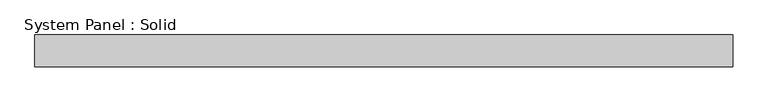
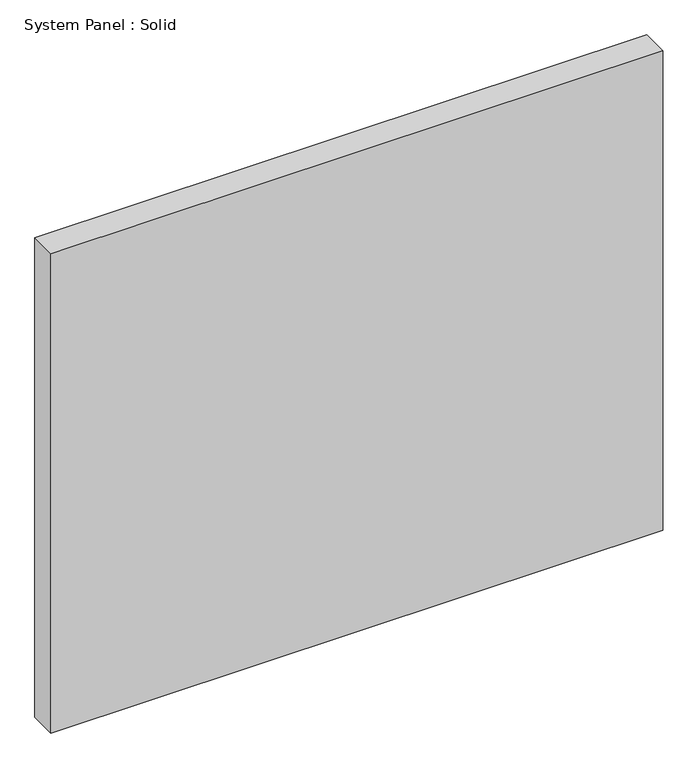
"""IFC4 building model written with IfcOpenShell, lengths in millimetres: plate geometry, System Panel : Solid."""

import ifcopenshell
import ifcopenshell.guid

model = None  # the IFC model being written
_history = None  # IfcOwnerHistory: only IFC2X3 demands one
_inside = {}  # id of a spatial element -> (the spatial element, [elements in it])
_under = {}  # id of a project, library or spatial element -> (it, [spatial elements below it])
_declared = {}  # id of a project -> (the project, [libraries it declares])
_typed = {}  # id of a type object -> (the type object, [elements of that type])
_made_of = {}  # id of a material, layer set ... -> (it, [elements and type objects made of it])


def new_model(schema):
    """Start an empty IFC model of exactly this schema.

    Asked for "IFC4X3", IfcOpenShell would pick the latest addendum, in which some entities
    have other attributes; the version numbers below select the first issue.
    IFC2X3 requires an IfcOwnerHistory on every rooted entity: one is made here for all.
    """
    global model, _history
    if schema == "IFC4X3":
        model = ifcopenshell.file(schema_version=(4, 3, 0, 0))
    else:
        model = ifcopenshell.file(schema=schema)
    _inside.clear()
    _under.clear()
    _declared.clear()
    _typed.clear()
    _made_of.clear()
    _history = None
    if model.schema == "IFC2X3":
        org = make("IfcOrganization", Name="unknown")
        user = make(
            "IfcPersonAndOrganization",
            ThePerson=make("IfcPerson", FamilyName="unknown"),
            TheOrganization=org,
        )
        app = make(
            "IfcApplication",
            ApplicationDeveloper=org,
            Version="unknown",
            ApplicationFullName="unknown",
            ApplicationIdentifier="unknown",
        )
        _history = make(
            "IfcOwnerHistory",
            OwningUser=user,
            OwningApplication=app,
            ChangeAction="ADDED",
            CreationDate=0,
        )
    return model


def make(cls, **values):
    """One entity of the class cls with the attributes given. An attribute that is None is left unset."""
    return model.create_entity(
        cls, **{name: value for name, value in values.items() if value is not None}
    )


def rooted(cls, **values):
    """An entity with a GlobalId (a new one), such as an element, a storey or a relation."""
    return make(cls, GlobalId=ifcopenshell.guid.new(), OwnerHistory=_history, **values)


def si_unit(unit_type, name, prefix=None):
    """IfcSIUnit, for example si_unit("LENGTHUNIT", "METRE", prefix="MILLI")."""
    return make("IfcSIUnit", UnitType=unit_type, Prefix=prefix, Name=name)


def assignment(units):
    """IfcUnitAssignment: the units of a project."""
    return None if units is None else make("IfcUnitAssignment", Units=units)


def point(xyz):
    """IfcCartesianPoint."""
    return None if xyz is None else make("IfcCartesianPoint", Coordinates=xyz)


def direction(xyz):
    """IfcDirection."""
    return None if xyz is None else make("IfcDirection", DirectionRatios=xyz)


def frame(location, z_axis=None, x_axis=None):
    """IfcAxis2Placement3D, a coordinate frame: its origin and axes. An axis left out is left unset."""
    return make(
        "IfcAxis2Placement3D",
        Location=point(location),
        Axis=direction(z_axis),
        RefDirection=direction(x_axis),
    )


def origin():
    """The frame at (0, 0, 0) with its axes left unset."""
    return frame((0.0, 0.0, 0.0))


def origin_with_axes():
    """The frame at (0, 0, 0) with the z axis (0, 0, 1) and the x axis (1, 0, 0) written out."""
    return frame((0.0, 0.0, 0.0), z_axis=(0.0, 0.0, 1.0), x_axis=(1.0, 0.0, 0.0))


def place(relative_to, where):
    """IfcLocalPlacement: puts the frame where relative to a parent placement (None: the world)."""
    return make(
        "IfcLocalPlacement", PlacementRelTo=relative_to, RelativePlacement=where
    )


def context(
    kind, dimensions, precision=None, world=None, true_north=None, identifier=None
):
    """IfcGeometricRepresentationContext, for example the 3D "Model" context."""
    return make(
        "IfcGeometricRepresentationContext",
        ContextIdentifier=identifier,
        ContextType=kind,
        CoordinateSpaceDimension=dimensions,
        Precision=precision,
        WorldCoordinateSystem=world,
        TrueNorth=true_north,
    )


def project(units=None, contexts=None):
    """IfcProject with its units and contexts."""
    return rooted(
        "IfcProject",
        Name="project",
        RepresentationContexts=contexts,
        UnitsInContext=assignment(units),
    )


def spatial(cls, under=None, at=None, **own):
    """A site, building, storey or space (cls), placed at a placement, below another one or the project."""
    s = rooted(cls, ObjectPlacement=at, **own)
    if under is not None:
        _under.setdefault(under.id(), (under, []))[1].append(s)
    return s


def polyline(points):
    """IfcPolyline through the points."""
    return make("IfcPolyline", Points=[point(p) for p in points])


def outline(outer, holes=None, kind="AREA"):
    """IfcArbitraryClosedProfileDef: a profile drawn as a closed curve; with holes, ...WithVoids."""
    if holes is None:
        return make("IfcArbitraryClosedProfileDef", ProfileType=kind, OuterCurve=outer)
    return make(
        "IfcArbitraryProfileDefWithVoids",
        ProfileType=kind,
        OuterCurve=outer,
        InnerCurves=holes,
    )


def extrude(swept, where, along, depth):
    """IfcExtrudedAreaSolid: the profile swept, set in the frame where, extruded along a direction by depth."""
    return make(
        "IfcExtrudedAreaSolid",
        SweptArea=swept,
        Position=where,
        ExtrudedDirection=direction(along),
        Depth=depth,
    )


def shape(context_of_items, identifier, shape_type, items):
    """IfcShapeRepresentation: the items that make up one representation, for example the "Body"."""
    return make(
        "IfcShapeRepresentation",
        ContextOfItems=context_of_items,
        RepresentationIdentifier=identifier,
        RepresentationType=shape_type,
        Items=items,
    )


def source(mapping_origin, context_of_items, identifier, shape_type, items):
    """IfcRepresentationMap: a shape defined once, which mapped items show again and again."""
    return make(
        "IfcRepresentationMap",
        MappingOrigin=mapping_origin,
        MappedRepresentation=shape(context_of_items, identifier, shape_type, items),
    )


def transform(
    local_origin,
    x_axis=None,
    y_axis=None,
    z_axis=None,
    scale=None,
    scale2=None,
    scale3=None,
    uniform=True,
):
    """IfcCartesianTransformationOperator3D, or its non-uniform kind. x_axis, y_axis, z_axis: its Axis1, 2, 3."""
    if uniform:
        return make(
            "IfcCartesianTransformationOperator3D",
            Axis1=direction(x_axis),
            Axis2=direction(y_axis),
            LocalOrigin=point(local_origin),
            Scale=scale,
            Axis3=direction(z_axis),
        )
    return make(
        "IfcCartesianTransformationOperator3DnonUniform",
        Axis1=direction(x_axis),
        Axis2=direction(y_axis),
        LocalOrigin=point(local_origin),
        Scale=scale,
        Axis3=direction(z_axis),
        Scale2=scale2,
        Scale3=scale3,
    )


def mapped(mapping_source, mapping_target):
    """IfcMappedItem: shows the shape of a source again, moved by a transform."""
    return make(
        "IfcMappedItem", MappingSource=mapping_source, MappingTarget=mapping_target
    )


def made_of(thing, what):
    """Note that an element or type object is made of a material, layer set ...; save() writes the relation."""
    if what is not None:
        _made_of.setdefault(what.id(), (what, []))[1].append(thing)
    return thing


def element(
    cls,
    number,
    at=None,
    inside=None,
    cuts=None,
    type_object=None,
    material=None,
    context=None,
    identifier="Body",
    shape_type=None,
    held_by="IfcProductDefinitionShape",
    body=None,
    shapes=None,
    **own,
):
    """One element of the class cls, such as IfcWall. Its Tag is "e" and its number.

    at: its placement. inside: the storey or other place that contains it. cuts: it is an
    opening in that element (IfcRelVoidsElement). A single representation is given by context,
    identifier, shape_type and body (its items); several are given by shapes. held_by: the class
    of the entity that holds the representations. save() writes the other relations.
    """
    e = rooted(cls, Tag="e%d" % number, ObjectPlacement=at, **own)
    if body is not None:
        shapes = [shape(context, identifier, shape_type, body)]
    if shapes is not None:
        e.Representation = make(held_by, Representations=shapes)
    if inside is not None:
        _inside.setdefault(inside.id(), (inside, []))[1].append(e)
    if cuts is not None:
        rooted(
            "IfcRelVoidsElement", RelatingBuildingElement=cuts, RelatedOpeningElement=e
        )
    if type_object is not None:
        _typed.setdefault(type_object.id(), (type_object, []))[1].append(e)
    return made_of(e, material)


def aggregate(whole, parts):
    """IfcRelAggregates: a whole, such as a stair, and the parts it consists of."""
    return rooted("IfcRelAggregates", RelatingObject=whole, RelatedObjects=parts)


def save(model, path):
    """Write the relations noted so far, then the file.

    IfcRelAggregates (storeys below a building ...), IfcRelContainedInSpatialStructure (elements
    in a storey), IfcRelDefinesByType, IfcRelAssociatesMaterial and IfcRelDeclares: one each for
    every whole, place, type object, material and project.
    """
    for whole, parts in _under.values():
        aggregate(whole, parts)
    for where, things in _inside.values():
        rooted(
            "IfcRelContainedInSpatialStructure",
            RelatedElements=things,
            RelatingStructure=where,
        )
    for kind, things in _typed.values():
        rooted("IfcRelDefinesByType", RelatedObjects=things, RelatingType=kind)
    for what, things in _made_of.values():
        rooted("IfcRelAssociatesMaterial", RelatedObjects=things, RelatingMaterial=what)
    for by, libraries in _declared.values():
        rooted("IfcRelDeclares", RelatingContext=by, RelatedDefinitions=libraries)
    model.write(path)


def system_panel_solid_8f383511(model_context):
    return source(origin(), model_context, "Body", "SweptSolid", [
        extrude(outline(polyline([(697.4416668, -19.05), (-697.4416668, -19.05), (-697.4416668, 44.45), (697.4416668, 44.45), (697.4416668, -19.05)])), origin_with_axes(), (0.0, 0.0, 1.0), 1155.7),
    ])


if __name__ == "__main__":
    model = new_model("IFC4")
    model_context = context("Model", 3, world=origin())
    ifc_project = project(units=[si_unit("LENGTHUNIT", "METRE", prefix="MILLI")], contexts=[model_context])
    site = spatial("IfcSite", under=ifc_project)
    building = spatial("IfcBuilding", under=site)
    placement = place(None, origin())
    system_panel_solid_shape = system_panel_solid_8f383511(model_context)
    element("IfcPlate", 1, ObjectType="System Panel : Solid", at=placement, inside=building, context=model_context, shape_type="MappedRepresentation", body=[
        mapped(system_panel_solid_shape, transform((0.0, 0.0, 0.0), x_axis=(1.0, 0.0, 0.0), y_axis=(0.0, 1.0, 0.0), z_axis=(0.0, 0.0, 1.0))),
    ])
    save(model, "model.ifc")

# Revit data of these elements
# Type "System Panel : Solid"
#   Construction Type Id = "MDOOR"
#   Analytic Construction = "Metal"
#   Visual Light Transmittance = 0
#   Solar Heat Gain Coefficient = 0
#   Heat Transfer Coefficient (U) = 0.651978 BTU/(h·ft²·°F)
#   Define Thermal Properties by = 1
# Element 1 (IfcPlate, "System Panel : Solid")
#   Materials on its faces: "Default"
# Materials
#   "Default": class "Miscellaneous", colour RGB 127 127 127, transparency 0, Cost = 0
